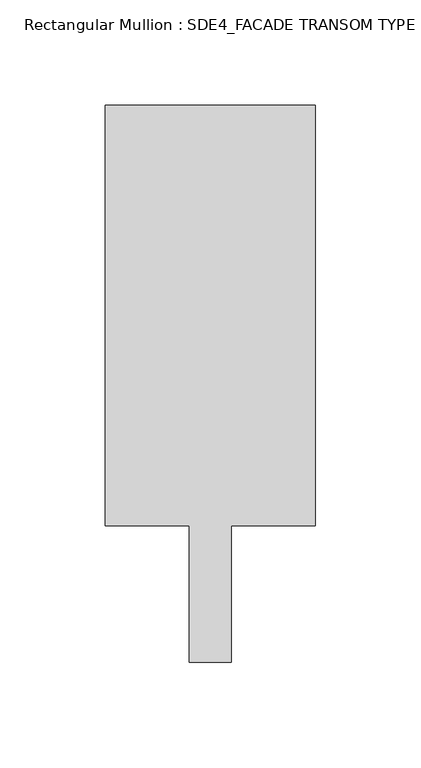
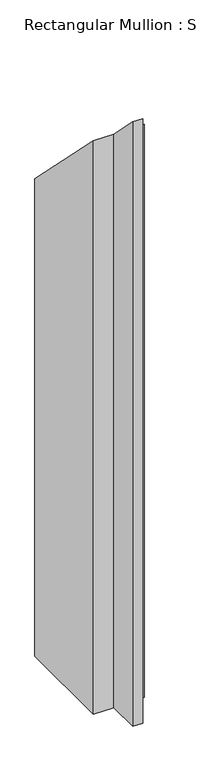
"""IFC4 building model written with IfcOpenShell, lengths in millimetres: member geometry, Rectangular Mullion : SDE4_FACADE TRANSOM TYPE 2."""

from ifc_helpers import new_model, si_unit, origin, place, context, project, spatial, faceted_brep, source, transform, mapped, element, save


def rectangular_mullion_sde4_facade_transom_type_2_b38f9d4b(model_context):
    return source(origin(), model_context, "Body", "Brep", [
        faceted_brep([(50.0, 132.5, -1129.375), (50.0, -67.5, -1129.375), (10.0, -67.5, -1129.375), (10.0, -132.5, -1129.375), (-10.0, -132.5, -1129.375), (-10.0, -67.5, -1129.375), (-50.0, -67.5, -1129.375), (-50.0, 132.5, -1129.375), (-50.0, 132.5, -132.5), (50.0, 132.5, -132.5), (-50.0, -67.5, 67.5), (-10.0, -67.5, 67.5), (-10.0, -132.5, 132.5), (10.0, -132.5, 132.5), (10.0, -67.5, 67.5), (50.0, -67.5, 67.5)], [[[0, 1, 2, 3, 4, 5, 6, 7]], [[8, 9, 0, 7]], [[10, 8, 7, 6]], [[11, 10, 6, 5]], [[12, 11, 5, 4]], [[13, 12, 4, 3]], [[14, 13, 3, 2]], [[15, 14, 2, 1]], [[9, 15, 1, 0]], [[9, 8, 10, 11, 12, 13, 14, 15]]]),
    ])


if __name__ == "__main__":
    model = new_model("IFC4")
    model_context = context("Model", 3, world=origin())
    ifc_project = project(units=[si_unit("LENGTHUNIT", "METRE", prefix="MILLI")], contexts=[model_context])
    site = spatial("IfcSite", under=ifc_project)
    building = spatial("IfcBuilding", under=site)
    placement = place(None, origin())
    rectangular_mullion_sde4_facade_transom_type_2_shape = rectangular_mullion_sde4_facade_transom_type_2_b38f9d4b(model_context)
    element("IfcMember", 1, ObjectType="Rectangular Mullion : SDE4_FACADE TRANSOM TYPE 2", at=placement, inside=building, context=model_context, shape_type="MappedRepresentation", body=[
        mapped(rectangular_mullion_sde4_facade_transom_type_2_shape, transform((0.0, 0.0, 0.0), x_axis=(1.0, 0.0, 0.0), y_axis=(0.0, 1.0, 0.0), z_axis=(0.0, 0.0, 1.0))),
    ])
    save(model, "model.ifc")

# Revit data of these elements
# Type "Rectangular Mullion : SDE4_FACADE TRANSOM TYPE 2"
#   built-in parameter 1007322 = 0.869423 (stored number, unit not read)
#   built-in parameter 1007321 = 0.164042 (stored number, unit not read)
#   built-in parameter 1007320 = 0.164042 (stored number, unit not read)
